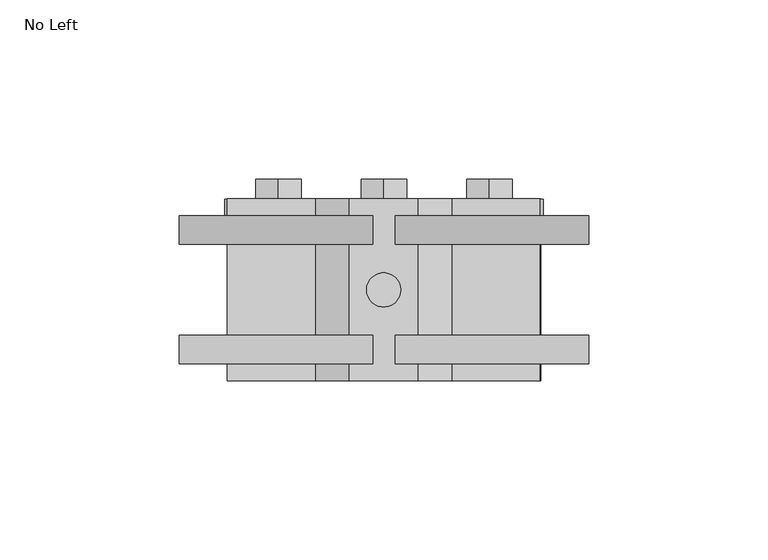
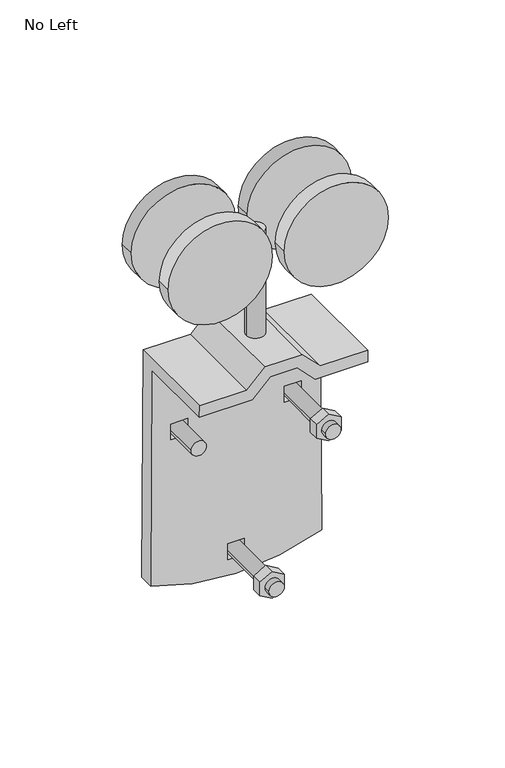
"""IFC4 building model written with IfcOpenShell, lengths in millimetres: proxy geometry, 087100_14 - Sliding and Folding Door Hardware - 5040 Box Rail Hangers : No Left."""

from ifc_helpers import new_model, si_unit, point, frame, frame_2d, origin, origin_with_axes, place, context, project, spatial, polyline, circle_curve, trimmed, segment, composite_curve, outline, extrude, source, transform, mapped, element, save
from ifc_brep_helpers import plane_surface, cylinder_surface, advanced_brep


def no_left_ff2eba34(model_context):
    return source(origin(), model_context, "Body", "SolidModel", [
        extrude(outline(polyline([(-117.3880521, -6.35), (-121.0542263, 0.0), (-117.3880521, 6.35), (-110.0557037, 6.35), (-106.3895295, 0.0), (-110.0557037, -6.35), (-117.3880521, -6.35)])), frame((0.0, -15.08125, 0.0), z_axis=(0.0, 1.0, 0.0), x_axis=(0.0, 0.0, 1.0)), (0.0, 0.0, 1.0), 5.55625),
        extrude(outline(polyline([(-110.0557037, -6.35), (-117.3880521, -6.35), (-121.0542263, 0.0), (-117.3880521, 6.35), (-110.0557037, 6.35), (-106.3895295, 0.0), (-110.0557037, -6.35)])), frame((0.0, 25.4, 0.0), z_axis=(0.0, 1.0, 0.0), x_axis=(0.0, 0.0, 1.0)), (0.0, 0.0, 1.0), 5.55625),
        extrude(outline(composite_curve([segment(trimmed(circle_curve(frame_2d((-113.7218779, 0.0)), 3.96875), [point((-113.7218779, -3.96875))], [point((-113.7218779, 3.96875))], False, "CARTESIAN"), True, "CONTINUOUS"), segment(trimmed(circle_curve(frame_2d((-113.7218779, 0.0)), 3.96875), [point((-113.7218779, 3.96875))], [point((-113.7218779, -3.96875))], False, "CARTESIAN"), True, "CONTINUOUS")], self_intersect=False)), frame((0.0, -19.05, 0.0), z_axis=(0.0, 1.0, 0.0), x_axis=(0.0, 0.0, 1.0)), (0.0, 0.0, 1.0), 44.45),
        extrude(outline(polyline([(-33.8196076, -35.8279106), (-41.151956, -35.8279106), (-44.8181303, -29.4779106), (-41.151956, -23.1279106), (-33.8196076, -23.1279106), (-30.1534334, -29.4779106), (-33.8196076, -35.8279106)])), frame((0.0, 25.4, 0.0), z_axis=(0.0, 1.0, 0.0), x_axis=(0.0, 0.0, 1.0)), (0.0, 0.0, 1.0), 5.55625),
        extrude(outline(composite_curve([segment(trimmed(circle_curve(frame_2d((-37.4857818, -29.4779106)), 3.96875), [point((-37.4857818, -33.4466606))], [point((-37.4857818, -25.5091606))], False, "CARTESIAN"), True, "CONTINUOUS"), segment(trimmed(circle_curve(frame_2d((-37.4857818, -29.4779106)), 3.96875), [point((-37.4857818, -25.5091606))], [point((-37.4857818, -33.4466606))], False, "CARTESIAN"), True, "CONTINUOUS")], self_intersect=False)), frame((0.0, 0.0, 0.0), z_axis=(0.0, 1.0, 0.0), x_axis=(0.0, 0.0, 1.0)), (0.0, 0.0, 1.0), 25.4),
        extrude(outline(polyline([(-41.151956, 23.1279765), (-44.8181303, 29.4779765), (-41.151956, 35.8279765), (-33.8196076, 35.8279765), (-30.1534334, 29.4779765), (-33.8196076, 23.1279765), (-41.151956, 23.1279765)])), frame((0.0, -15.08125, 0.0), z_axis=(0.0, 1.0, 0.0), x_axis=(0.0, 0.0, 1.0)), (0.0, 0.0, 1.0), 5.55625),
        extrude(outline(polyline([(-33.8196076, 23.1279765), (-41.151956, 23.1279765), (-44.8181303, 29.4779765), (-41.151956, 35.8279765), (-33.8196076, 35.8279765), (-30.1534334, 29.4779765), (-33.8196076, 23.1279765)])), frame((0.0, 25.4, 0.0), z_axis=(0.0, 1.0, 0.0), x_axis=(0.0, 0.0, 1.0)), (0.0, 0.0, 1.0), 5.55625),
        extrude(outline(composite_curve([segment(trimmed(circle_curve(frame_2d((-37.4857818, 29.4779765)), 3.96875), [point((-37.4857818, 25.5092265))], [point((-37.4857818, 33.4467265))], False, "CARTESIAN"), True, "CONTINUOUS"), segment(trimmed(circle_curve(frame_2d((-37.4857818, 29.4779765)), 3.96875), [point((-37.4857818, 33.4467265))], [point((-37.4857818, 25.5092265))], False, "CARTESIAN"), True, "CONTINUOUS")], self_intersect=False)), frame((0.0, -19.05, 0.0), z_axis=(0.0, 1.0, 0.0), x_axis=(0.0, 0.0, 1.0)), (0.0, 0.0, 1.0), 44.45),
        advanced_brep(
        [(-44.4707374, 25.4, -118.5726247), (-43.7119983, 25.4, 6.35), (-19.059057, 25.4, 6.35), (-9.6566784, 25.4, 15.7523786), (9.6563712, 25.4, 15.7523786), (19.0589621, 25.4, 6.35), (43.7118564, 25.4, 6.35), (44.4707374, 25.4, -118.5726247), (-25.119743, 25.4, -33.1275483), (-33.8360782, 25.4, -33.1275483), (-33.8360782, 25.4, -41.8440154), (-25.119743, 25.4, -41.8440154), (33.8360782, 25.4, -33.1275483), (25.1198748, 25.4, -33.1275483), (25.1198748, 25.4, -41.8440154), (33.8360782, 25.4, -41.8440154), (4.3581017, 25.4, -109.3636444), (-4.3581017, 25.4, -109.3636444), (-4.3581017, 25.4, -118.0801114), (4.3581017, 25.4, -118.0801114), (-43.7119983, -25.4, 6.35), (-43.7505662, -25.4, 0.0), (-16.4288009, -25.4, 0.0), (-7.0264223, -25.4, 9.4023786), (7.0261571, -25.4, 9.4023786), (16.428748, -25.4, 0.0), (43.7504315, -25.4, 0.0), (43.7118564, -25.4, 6.35), (19.0589621, -25.4, 6.35), (9.6563712, -25.4, 15.7523786), (-9.6566784, -25.4, 15.7523786), (-19.059057, -25.4, 6.35), (-44.4707374, 17.4625, -118.5726247), (-43.7505662, 17.4625, 0.0), (-16.4288009, 17.4625, 0.0), (-7.0264223, 17.4625, 9.4023786), (7.0261571, 17.4625, 9.4023786), (16.428748, 17.4625, 0.0), (43.7504315, 17.4625, 0.0), (44.4707374, 17.4625, -118.5726247), (19.0589621, 17.4625, 6.35), (9.6563712, 17.4625, 15.7523786), (-9.6566784, 17.4625, 15.7523786), (-19.059057, 17.4625, 6.35), (-25.119743, 17.4625, -33.1275483), (-25.119743, 17.4625, -41.8440154), (-33.8360782, 17.4625, -41.8440154), (-33.8360782, 17.4625, -33.1275483), (33.8360782, 17.4625, -33.1275483), (33.8360782, 17.4625, -41.8440154), (25.1198748, 17.4625, -41.8440154), (25.1198748, 17.4625, -33.1275483), (4.3581017, 17.4625, -109.3636444), (4.3581017, 17.4625, -118.0801114), (-4.3581017, 17.4625, -118.0801114), (-4.3581017, 17.4625, -109.3636444)],
        [
            (0, 1),
            (1, 2),
            (2, 3),
            (3, 4),
            (4, 5),
            (5, 6),
            (6, 7),
            (7, 0, circle_curve(frame((0.0, 25.4, -6.3557626), z_axis=(0.0, 1.0, 0.0), x_axis=(1.0, 0.0, 0.0)), 120.7073761)),
            (8, 9),
            (9, 10),
            (10, 11),
            (11, 8),
            (12, 13),
            (13, 14),
            (14, 15),
            (15, 12),
            (16, 17),
            (17, 18),
            (18, 19),
            (19, 16),
            (20, 21),
            (21, 22),
            (22, 23),
            (23, 24),
            (24, 25),
            (25, 26),
            (26, 27),
            (27, 28),
            (28, 29),
            (29, 30),
            (30, 31),
            (31, 20),
            (0, 32),
            (32, 33),
            (33, 21),
            (20, 1),
            (33, 34),
            (34, 22),
            (34, 35),
            (35, 23),
            (35, 36),
            (36, 24),
            (36, 37),
            (37, 25),
            (37, 38),
            (38, 26),
            (6, 27),
            (38, 39),
            (39, 7),
            (5, 40),
            (40, 28),
            (4, 41),
            (41, 29),
            (3, 42),
            (42, 30),
            (2, 43),
            (43, 31),
            (32, 39, circle_curve(frame((0.0, 17.4625, -6.3557626), z_axis=(0.0, -1.0, 0.0), x_axis=(1.0, 0.0, 0.0)), 120.7073761)),
            (44, 45),
            (45, 46),
            (46, 47),
            (47, 44),
            (48, 49),
            (49, 50),
            (50, 51),
            (51, 48),
            (52, 53),
            (53, 54),
            (54, 55),
            (55, 52),
            (11, 45),
            (44, 8),
            (10, 46),
            (9, 47),
            (15, 49),
            (48, 12),
            (14, 50),
            (13, 51),
            (19, 53),
            (52, 16),
            (18, 54),
            (17, 55),
        ],
        [
            plane_surface(frame((-46.969086, 25.4, -529.9133004), z_axis=(0.0, 1.0, 0.0), x_axis=(-0.006073560512695754, 0.0, -0.9999815557612544))),
            plane_surface(frame((-46.969086, -25.4, -529.9133004), z_axis=(0.0, -1.0, 0.0), x_axis=(0.006073560512695754, 0.0, 0.9999815557612544))),
            plane_surface(frame((-43.7119983, 25.4, 6.35), z_axis=(-0.9999815557612544, 0.0, 0.006073560512695754), x_axis=(0.0, -1.0, 0.0))),
            plane_surface(frame((-43.7505662, 25.4, 0.0), z_axis=(0.0, 0.0, -1.0), x_axis=(0.0, -1.0, 0.0))),
            plane_surface(frame((-16.4288009, 25.4, 0.0), z_axis=(0.7071067811865476, 0.0, -0.7071067811865476), x_axis=(0.0, -1.0, 0.0))),
            plane_surface(frame((-7.0264223, 25.4, 9.4023786), z_axis=(0.0, 0.0, -1.0), x_axis=(0.0, -1.0, 0.0))),
            plane_surface(frame((7.0261571, 25.4, 9.4023786), z_axis=(-0.7070987963768838, 0.0, -0.7071147659060459), x_axis=(0.0, -1.0, 0.0))),
            plane_surface(frame((16.428748, 25.4, 0.0), z_axis=(0.0, 0.0, -1.0), x_axis=(0.0, -1.0, 0.0))),
            plane_surface(frame((43.7504315, 25.4, 0.0), z_axis=(0.9999815488618892, 0.0, 0.006074696352680505), x_axis=(0.0, -1.0, 0.0))),
            plane_surface(frame((43.7118564, 25.4, 6.35), z_axis=(0.0, 0.0, 1.0), x_axis=(0.0, -1.0, 0.0))),
            plane_surface(frame((19.0589621, 25.4, 6.35), z_axis=(0.7070987963768809, 0.0, 0.7071147659060488), x_axis=(0.0, -1.0, 0.0))),
            plane_surface(frame((9.6563712, 25.4, 15.7523786), z_axis=(0.0, 0.0, 1.0), x_axis=(0.0, -1.0, 0.0))),
            plane_surface(frame((-9.6566784, 25.4, 15.7523786), z_axis=(-0.7071067811865457, 0.0, 0.7071067811865495), x_axis=(0.0, -1.0, 0.0))),
            plane_surface(frame((-19.059057, 25.4, 6.35), z_axis=(0.0, 0.0, 1.0), x_axis=(0.0, -1.0, 0.0))),
            plane_surface(frame((-46.969086, 17.4625, -529.9133004), z_axis=(0.0, -1.0, 0.0), x_axis=(0.006073560512693812, 0.0, 0.9999815557612544))),
            cylinder_surface(frame((0.0, 17.4625, -6.3557626), z_axis=(0.0, 1.0, 0.0), x_axis=(1.0, 0.0, 0.0)), 120.7073761),
            plane_surface(frame((-25.119743, 25.4, -33.1275483), z_axis=(-1.0, 0.0, 0.0), x_axis=(0.0, -1.0, 0.0))),
            plane_surface(frame((-25.119743, 25.4, -41.8440154), z_axis=(0.0, 0.0, 1.0), x_axis=(0.0, -1.0, 0.0))),
            plane_surface(frame((-33.8360782, 25.4, -41.8440154), z_axis=(1.0, 0.0, 0.0), x_axis=(0.0, -1.0, 0.0))),
            plane_surface(frame((-33.8360782, 25.4, -33.1275483), z_axis=(0.0, 0.0, -1.0), x_axis=(0.0, -1.0, 0.0))),
            plane_surface(frame((33.8360782, 25.4, -33.1275483), z_axis=(-1.0, 0.0, 0.0), x_axis=(0.0, -1.0, 0.0))),
            plane_surface(frame((33.8360782, 25.4, -41.8440154), z_axis=(0.0, 0.0, 1.0), x_axis=(0.0, -1.0, 0.0))),
            plane_surface(frame((25.1198748, 25.4, -41.8440154), z_axis=(1.0, 0.0, 0.0), x_axis=(0.0, -1.0, 0.0))),
            plane_surface(frame((25.1198748, 25.4, -33.1275483), z_axis=(0.0, 0.0, -1.0), x_axis=(0.0, -1.0, 0.0))),
            plane_surface(frame((4.3581017, 25.4, -109.3636444), z_axis=(-1.0, 0.0, 0.0), x_axis=(0.0, -1.0, 0.0))),
            plane_surface(frame((4.3581017, 25.4, -118.0801114), z_axis=(0.0, 0.0, 1.0), x_axis=(0.0, -1.0, 0.0))),
            plane_surface(frame((-4.3581017, 25.4, -118.0801114), z_axis=(1.0, 0.0, 0.0), x_axis=(0.0, -1.0, 0.0))),
            plane_surface(frame((-4.3581017, 25.4, -109.3636444), z_axis=(0.0, 0.0, -1.0), x_axis=(0.0, -1.0, 0.0))),
        ],
        [
            (0, [[1, 2, 3, 4, 5, 6, 7, 8], [9, 10, 11, 12], [13, 14, 15, 16], [17, 18, 19, 20]]),
            (1, [[21, 22, 23, 24, 25, 26, 27, 28, 29, 30, 31, 32]]),
            (2, [[33, 34, 35, -21, 36, -1]]),
            (3, [[-35, 37, 38, -22]]),
            (4, [[-38, 39, 40, -23]]),
            (5, [[-40, 41, 42, -24]]),
            (6, [[-42, 43, 44, -25]]),
            (7, [[-44, 45, 46, -26]]),
            (8, [[47, -27, -46, 48, 49, -7]]),
            (9, [[50, 51, -28, -47, -6]]),
            (10, [[52, 53, -29, -51, -50, -5]]),
            (11, [[54, 55, -30, -53, -52, -4]]),
            (12, [[56, 57, -31, -55, -54, -3]]),
            (13, [[-32, -57, -56, -2, -36]]),
            (14, [[-48, -45, -43, -41, -39, -37, -34, 58], [59, 60, 61, 62], [63, 64, 65, 66], [67, 68, 69, 70]]),
            (15, [[-49, -58, -33, -8]]),
            (16, [[71, -59, 72, -12]]),
            (17, [[73, -60, -71, -11]]),
            (18, [[74, -61, -73, -10]]),
            (19, [[-72, -62, -74, -9]]),
            (20, [[75, -63, 76, -16]]),
            (21, [[77, -64, -75, -15]]),
            (22, [[78, -65, -77, -14]]),
            (23, [[-76, -66, -78, -13]]),
            (24, [[79, -67, 80, -20]]),
            (25, [[81, -68, -79, -19]]),
            (26, [[82, -69, -81, -18]]),
            (27, [[-80, -70, -82, -17]]),
        ],
    ),
        extrude(outline(composite_curve([segment(trimmed(circle_curve(frame_2d((71.8251107, -30.1481535)), 27.0838855), [point((71.8251107, -57.232039))], [point((71.8251107, -3.0642681))], False, "CARTESIAN"), True, "CONTINUOUS"), segment(trimmed(circle_curve(frame_2d((71.8251107, -30.1481535)), 27.0838855), [point((71.8251107, -3.0642681))], [point((71.8251107, -57.232039))], False, "CARTESIAN"), True, "CONTINUOUS")], self_intersect=False)), frame((0.0, -20.6375, 0.0), z_axis=(0.0, 1.0, 0.0), x_axis=(0.0, 0.0, 1.0)), (0.0, 0.0, 1.0), 7.9375),
        extrude(outline(composite_curve([segment(trimmed(circle_curve(frame_2d((71.8251107, 30.2054611)), 27.0838855), [point((71.8251107, 3.1215756))], [point((71.8251107, 57.2893465))], False, "CARTESIAN"), True, "CONTINUOUS"), segment(trimmed(circle_curve(frame_2d((71.8251107, 30.2054611)), 27.0838855), [point((71.8251107, 57.2893465))], [point((71.8251107, 3.1215756))], False, "CARTESIAN"), True, "CONTINUOUS")], self_intersect=False)), frame((0.0, -20.6375, 0.0), z_axis=(0.0, 1.0, 0.0), x_axis=(0.0, 0.0, 1.0)), (0.0, 0.0, 1.0), 7.9375),
        extrude(outline(composite_curve([segment(trimmed(circle_curve(frame_2d((-0.0657734, 0.0)), 4.7625), [point((-4.8282734, 0.0))], [point((4.6967266, 0.0))], False, "CARTESIAN"), True, "CONTINUOUS"), segment(trimmed(circle_curve(frame_2d((-0.0657734, 0.0)), 4.7625), [point((4.6967266, 0.0))], [point((-4.8282734, 0.0))], False, "CARTESIAN"), True, "CONTINUOUS")], self_intersect=False)), origin_with_axes(), (0.0, 0.0, 1.0), 73.5534737),
        extrude(outline(composite_curve([segment(trimmed(circle_curve(frame_2d((71.8251107, -30.1481535)), 27.0838855), [point((71.8251107, -57.232039))], [point((71.8251107, -3.0642681))], False, "CARTESIAN"), True, "CONTINUOUS"), segment(trimmed(circle_curve(frame_2d((71.8251107, -30.1481535)), 27.0838855), [point((71.8251107, -3.0642681))], [point((71.8251107, -57.232039))], False, "CARTESIAN"), True, "CONTINUOUS")], self_intersect=False)), frame((0.0, 12.7, 0.0), z_axis=(0.0, 1.0, 0.0), x_axis=(0.0, 0.0, 1.0)), (0.0, 0.0, 1.0), 7.9375),
        extrude(outline(composite_curve([segment(trimmed(circle_curve(frame_2d((71.8251107, 30.2054611)), 27.0838855), [point((71.8251107, 3.1215756))], [point((71.8251107, 57.2893465))], False, "CARTESIAN"), True, "CONTINUOUS"), segment(trimmed(circle_curve(frame_2d((71.8251107, 30.2054611)), 27.0838855), [point((71.8251107, 57.2893465))], [point((71.8251107, 3.1215756))], False, "CARTESIAN"), True, "CONTINUOUS")], self_intersect=False)), frame((0.0, 12.7, 0.0), z_axis=(0.0, 1.0, 0.0), x_axis=(0.0, 0.0, 1.0)), (0.0, 0.0, 1.0), 7.9375),
    ])


if __name__ == "__main__":
    model = new_model("IFC4")
    model_context = context("Model", 3, world=origin())
    ifc_project = project(units=[si_unit("LENGTHUNIT", "METRE", prefix="MILLI")], contexts=[model_context])
    site = spatial("IfcSite", under=ifc_project)
    building = spatial("IfcBuilding", under=site)
    placement = place(None, origin())
    no_left_shape = no_left_ff2eba34(model_context)
    element("IfcBuildingElementProxy", 1, Name="087100_14 - Sliding and Folding Door Hardware - 5040 Box Rail Hangers : No Left", ObjectType="087100_14 - Sliding and Folding Door Hardware - 5040 Box Rail Hangers : No Left", at=placement, inside=building, context=model_context, shape_type="MappedRepresentation", body=[
        mapped(no_left_shape, transform((0.0, 0.0, 0.0), x_axis=(1.0, 0.0, 0.0), y_axis=(0.0, 1.0, 0.0), z_axis=(0.0, 0.0, 1.0))),
    ])
    save(model, "model.ifc")

# Revit data of these elements
# Type "087100_14 - Sliding and Folding Door Hardware - 5040 Box Rail Hangers : No Left"
#   Default Elevation = 4' - 0"
#   Left Bolt = element 2408421
#   Bracket Material = BOX RAIL HANGER W/ GALV. FASTNERS (NATIONAL 5040)
#   Bottom Bolt = element 2408420
# Element 1 (IfcBuildingElementProxy, "087100_14 - Sliding and Folding Door Hardware - 5040 Box Rail Hangers : No Left")
#   Materials on its faces: "STRUCTURAL BOLTS (PAINT TO MATCH STEEL FINISH)", "BOX RAIL HANGER W/ GALV. FASTNERS (NATIONAL 5040)"
# Materials
#   "BOX RAIL HANGER W/ GALV. FASTNERS (NATIONAL 5040)": class "Metal", colour RGB 199 199 199, transparency 0, Description = "Structural steel, ASTM A36 Grade B, mill finish", Cost = 0
#   "STRUCTURAL BOLTS (PAINT TO MATCH STEEL FINISH)": class "Generic", colour RGB 120 120 120, transparency 0, Cost = 0
